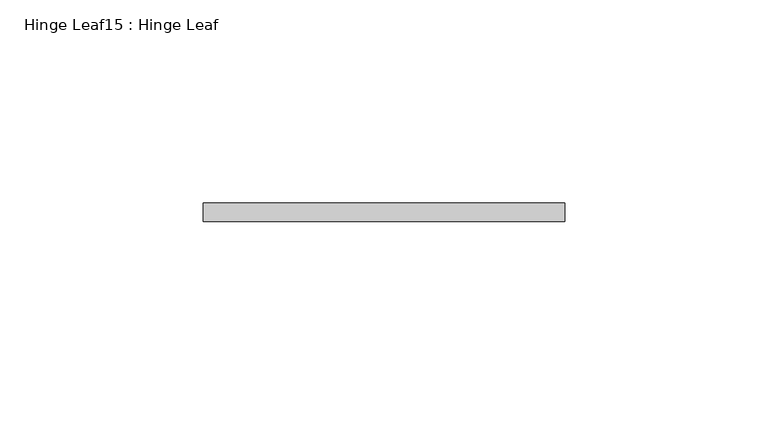
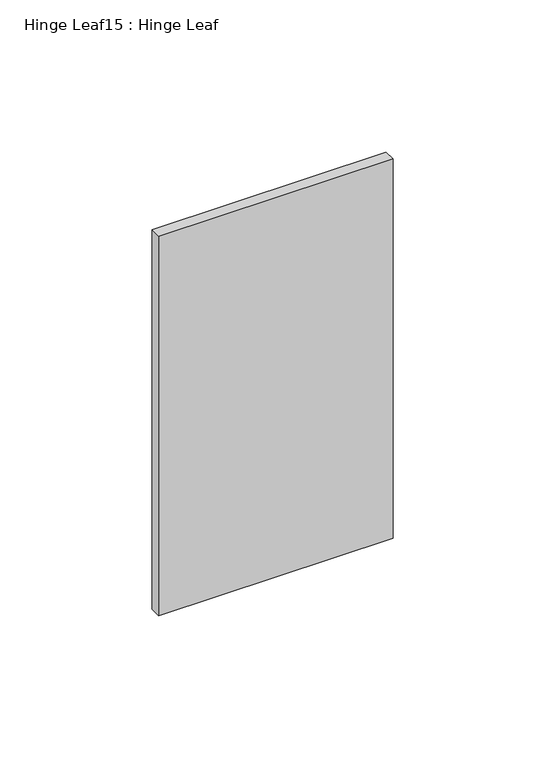
"""IFC4 building model written with IfcOpenShell, lengths in millimetres: proxy geometry, Hinge Leaf15 : Hinge Leaf."""

from ifc_helpers import new_model, si_unit, frame, origin, place, context, project, spatial, polyline, outline, extrude, source, transform, mapped, element, save


def hinge_leaf15_hinge_leaf_b84fefac(model_context):
    return source(origin(), model_context, "Body", "SweptSolid", [
        extrude(outline(polyline([(587327.7934739, -534096.6663841), (587416.6934739, -534096.6663841), (587416.6934739, -534101.2383841), (587327.7934739, -534101.2383841), (587327.7934739, -534096.6663841)])), frame((0.0, 0.0, 311.15), z_axis=(0.0, 0.0, 1.0), x_axis=(1.0, 0.0, 0.0)), (0.0, 0.0, 1.0), 152.4),
    ])


if __name__ == "__main__":
    model = new_model("IFC4")
    model_context = context("Model", 3, world=origin())
    ifc_project = project(units=[si_unit("LENGTHUNIT", "METRE", prefix="MILLI")], contexts=[model_context])
    site = spatial("IfcSite", under=ifc_project)
    building = spatial("IfcBuilding", under=site)
    placement = place(None, origin())
    hinge_leaf15_hinge_leaf_shape = hinge_leaf15_hinge_leaf_b84fefac(model_context)
    element("IfcBuildingElementProxy", 1, Name="Hinge Leaf15 : Hinge Leaf", ObjectType="Hinge Leaf15 : Hinge Leaf", at=placement, inside=building, context=model_context, shape_type="MappedRepresentation", body=[
        mapped(hinge_leaf15_hinge_leaf_shape, transform((0.0, 0.0, 0.0), x_axis=(1.0, 0.0, 0.0), y_axis=(0.0, 1.0, 0.0), z_axis=(0.0, 0.0, 1.0))),
    ])
    save(model, "model.ifc")

# Revit data of these elements
# Element 1 (IfcBuildingElementProxy, "Hinge Leaf15 : Hinge Leaf")
#   Materials on its faces: "6\"X6\" WELD-ON STL BUTT HINGE"
# Materials
#   "6\"X6\" WELD-ON STL BUTT HINGE": class "Metal", colour RGB 189 187 185, transparency 0, Description = "Carbon steel", Cost = 0
